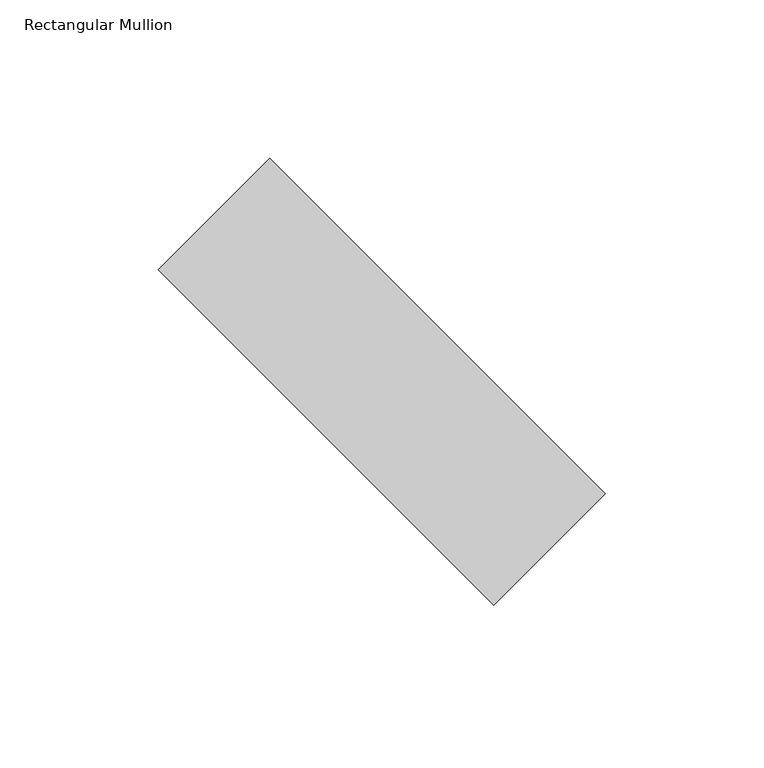
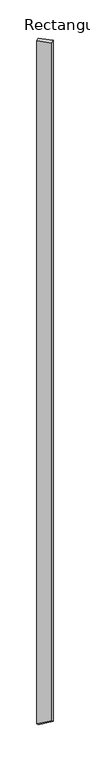
"""IFC4 building model written with IfcOpenShell, lengths in millimetres: member geometry, Rectangular Mullion : tilted mullions."""

import ifcopenshell
import ifcopenshell.guid

model = None  # the IFC model being written
_history = None  # IfcOwnerHistory: only IFC2X3 demands one
_inside = {}  # id of a spatial element -> (the spatial element, [elements in it])
_under = {}  # id of a project, library or spatial element -> (it, [spatial elements below it])
_declared = {}  # id of a project -> (the project, [libraries it declares])
_typed = {}  # id of a type object -> (the type object, [elements of that type])
_made_of = {}  # id of a material, layer set ... -> (it, [elements and type objects made of it])


def new_model(schema):
    """Start an empty IFC model of exactly this schema.

    Asked for "IFC4X3", IfcOpenShell would pick the latest addendum, in which some entities
    have other attributes; the version numbers below select the first issue.
    IFC2X3 requires an IfcOwnerHistory on every rooted entity: one is made here for all.
    """
    global model, _history
    if schema == "IFC4X3":
        model = ifcopenshell.file(schema_version=(4, 3, 0, 0))
    else:
        model = ifcopenshell.file(schema=schema)
    _inside.clear()
    _under.clear()
    _declared.clear()
    _typed.clear()
    _made_of.clear()
    _history = None
    if model.schema == "IFC2X3":
        org = make("IfcOrganization", Name="unknown")
        user = make(
            "IfcPersonAndOrganization",
            ThePerson=make("IfcPerson", FamilyName="unknown"),
            TheOrganization=org,
        )
        app = make(
            "IfcApplication",
            ApplicationDeveloper=org,
            Version="unknown",
            ApplicationFullName="unknown",
            ApplicationIdentifier="unknown",
        )
        _history = make(
            "IfcOwnerHistory",
            OwningUser=user,
            OwningApplication=app,
            ChangeAction="ADDED",
            CreationDate=0,
        )
    return model


def make(cls, **values):
    """One entity of the class cls with the attributes given. An attribute that is None is left unset."""
    return model.create_entity(
        cls, **{name: value for name, value in values.items() if value is not None}
    )


def rooted(cls, **values):
    """An entity with a GlobalId (a new one), such as an element, a storey or a relation."""
    return make(cls, GlobalId=ifcopenshell.guid.new(), OwnerHistory=_history, **values)


def si_unit(unit_type, name, prefix=None):
    """IfcSIUnit, for example si_unit("LENGTHUNIT", "METRE", prefix="MILLI")."""
    return make("IfcSIUnit", UnitType=unit_type, Prefix=prefix, Name=name)


def assignment(units):
    """IfcUnitAssignment: the units of a project."""
    return None if units is None else make("IfcUnitAssignment", Units=units)


def point(xyz):
    """IfcCartesianPoint."""
    return None if xyz is None else make("IfcCartesianPoint", Coordinates=xyz)


def direction(xyz):
    """IfcDirection."""
    return None if xyz is None else make("IfcDirection", DirectionRatios=xyz)


def frame(location, z_axis=None, x_axis=None):
    """IfcAxis2Placement3D, a coordinate frame: its origin and axes. An axis left out is left unset."""
    return make(
        "IfcAxis2Placement3D",
        Location=point(location),
        Axis=direction(z_axis),
        RefDirection=direction(x_axis),
    )


def origin():
    """The frame at (0, 0, 0) with its axes left unset."""
    return frame((0.0, 0.0, 0.0))


def place(relative_to, where):
    """IfcLocalPlacement: puts the frame where relative to a parent placement (None: the world)."""
    return make(
        "IfcLocalPlacement", PlacementRelTo=relative_to, RelativePlacement=where
    )


def context(
    kind, dimensions, precision=None, world=None, true_north=None, identifier=None
):
    """IfcGeometricRepresentationContext, for example the 3D "Model" context."""
    return make(
        "IfcGeometricRepresentationContext",
        ContextIdentifier=identifier,
        ContextType=kind,
        CoordinateSpaceDimension=dimensions,
        Precision=precision,
        WorldCoordinateSystem=world,
        TrueNorth=true_north,
    )


def project(units=None, contexts=None):
    """IfcProject with its units and contexts."""
    return rooted(
        "IfcProject",
        Name="project",
        RepresentationContexts=contexts,
        UnitsInContext=assignment(units),
    )


def spatial(cls, under=None, at=None, **own):
    """A site, building, storey or space (cls), placed at a placement, below another one or the project."""
    s = rooted(cls, ObjectPlacement=at, **own)
    if under is not None:
        _under.setdefault(under.id(), (under, []))[1].append(s)
    return s


def faces_of(points, faces, orient=None, outer=None):
    """IfcFace entities. A face is a list of loops; a loop is a list of indices into points, from 0.

    orient and outer hold one flag for each loop. By default every Orientation is true, the
    first loop of a face is its IfcFaceOuterBound and the others are IfcFaceBound.
    """
    made = []
    for i, loops in enumerate(faces):
        bounds = []
        for j, loop in enumerate(loops):
            is_outer = j == 0 if outer is None else outer[i][j]
            bounds.append(
                make(
                    "IfcFaceOuterBound" if is_outer else "IfcFaceBound",
                    Bound=make("IfcPolyLoop", Polygon=[points[k] for k in loop]),
                    Orientation=True if orient is None else orient[i][j],
                )
            )
        made.append(make("IfcFace", Bounds=bounds))
    return made


def faceted_brep(points, faces, orient=None, outer=None, voids=None):
    """IfcFacetedBrep: a solid bounded by flat faces; with voids (closed shells), ...WithVoids."""
    shared = [point(p) for p in points]
    hull = make("IfcClosedShell", CfsFaces=faces_of(shared, faces, orient, outer))
    if voids is None:
        return make("IfcFacetedBrep", Outer=hull)
    return make(
        "IfcFacetedBrepWithVoids",
        Outer=hull,
        Voids=[
            make(cls, CfsFaces=faces_of(shared, fs, o, b)) for cls, fs, o, b in voids
        ],
    )


def shape(context_of_items, identifier, shape_type, items):
    """IfcShapeRepresentation: the items that make up one representation, for example the "Body"."""
    return make(
        "IfcShapeRepresentation",
        ContextOfItems=context_of_items,
        RepresentationIdentifier=identifier,
        RepresentationType=shape_type,
        Items=items,
    )


def source(mapping_origin, context_of_items, identifier, shape_type, items):
    """IfcRepresentationMap: a shape defined once, which mapped items show again and again."""
    return make(
        "IfcRepresentationMap",
        MappingOrigin=mapping_origin,
        MappedRepresentation=shape(context_of_items, identifier, shape_type, items),
    )


def transform(
    local_origin,
    x_axis=None,
    y_axis=None,
    z_axis=None,
    scale=None,
    scale2=None,
    scale3=None,
    uniform=True,
):
    """IfcCartesianTransformationOperator3D, or its non-uniform kind. x_axis, y_axis, z_axis: its Axis1, 2, 3."""
    if uniform:
        return make(
            "IfcCartesianTransformationOperator3D",
            Axis1=direction(x_axis),
            Axis2=direction(y_axis),
            LocalOrigin=point(local_origin),
            Scale=scale,
            Axis3=direction(z_axis),
        )
    return make(
        "IfcCartesianTransformationOperator3DnonUniform",
        Axis1=direction(x_axis),
        Axis2=direction(y_axis),
        LocalOrigin=point(local_origin),
        Scale=scale,
        Axis3=direction(z_axis),
        Scale2=scale2,
        Scale3=scale3,
    )


def mapped(mapping_source, mapping_target):
    """IfcMappedItem: shows the shape of a source again, moved by a transform."""
    return make(
        "IfcMappedItem", MappingSource=mapping_source, MappingTarget=mapping_target
    )


def made_of(thing, what):
    """Note that an element or type object is made of a material, layer set ...; save() writes the relation."""
    if what is not None:
        _made_of.setdefault(what.id(), (what, []))[1].append(thing)
    return thing


def element(
    cls,
    number,
    at=None,
    inside=None,
    cuts=None,
    type_object=None,
    material=None,
    context=None,
    identifier="Body",
    shape_type=None,
    held_by="IfcProductDefinitionShape",
    body=None,
    shapes=None,
    **own,
):
    """One element of the class cls, such as IfcWall. Its Tag is "e" and its number.

    at: its placement. inside: the storey or other place that contains it. cuts: it is an
    opening in that element (IfcRelVoidsElement). A single representation is given by context,
    identifier, shape_type and body (its items); several are given by shapes. held_by: the class
    of the entity that holds the representations. save() writes the other relations.
    """
    e = rooted(cls, Tag="e%d" % number, ObjectPlacement=at, **own)
    if body is not None:
        shapes = [shape(context, identifier, shape_type, body)]
    if shapes is not None:
        e.Representation = make(held_by, Representations=shapes)
    if inside is not None:
        _inside.setdefault(inside.id(), (inside, []))[1].append(e)
    if cuts is not None:
        rooted(
            "IfcRelVoidsElement", RelatingBuildingElement=cuts, RelatedOpeningElement=e
        )
    if type_object is not None:
        _typed.setdefault(type_object.id(), (type_object, []))[1].append(e)
    return made_of(e, material)


def aggregate(whole, parts):
    """IfcRelAggregates: a whole, such as a stair, and the parts it consists of."""
    return rooted("IfcRelAggregates", RelatingObject=whole, RelatedObjects=parts)


def save(model, path):
    """Write the relations noted so far, then the file.

    IfcRelAggregates (storeys below a building ...), IfcRelContainedInSpatialStructure (elements
    in a storey), IfcRelDefinesByType, IfcRelAssociatesMaterial and IfcRelDeclares: one each for
    every whole, place, type object, material and project.
    """
    for whole, parts in _under.values():
        aggregate(whole, parts)
    for where, things in _inside.values():
        rooted(
            "IfcRelContainedInSpatialStructure",
            RelatedElements=things,
            RelatingStructure=where,
        )
    for kind, things in _typed.values():
        rooted("IfcRelDefinesByType", RelatedObjects=things, RelatingType=kind)
    for what, things in _made_of.values():
        rooted("IfcRelAssociatesMaterial", RelatedObjects=things, RelatingMaterial=what)
    for by, libraries in _declared.values():
        rooted("IfcRelDeclares", RelatingContext=by, RelatedDefinitions=libraries)
    model.write(path)


def rectangular_mullion_71da9a33(model_context):
    return source(origin(), model_context, "Body", "Brep", [
        faceted_brep([(-35.3553391, 70.7106781, 0.0), (-70.7106781, 35.3553391, 0.0), (35.3553391, -70.7106781, 0.0), (70.7106781, -35.3553391, 0.0), (-35.3553391, 70.7106781, -8054.4890214), (-70.7106781, 35.3553391, -8009.469781), (35.3553391, -70.7106781, -7944.2056108), (70.7106781, -35.3553391, -7989.2248513)], [[[0, 1, 2, 3]], [[1, 0, 4, 5]], [[2, 1, 5, 6]], [[3, 2, 6, 7]], [[0, 3, 7, 4]], [[4, 7, 6, 5]]]),
    ])


if __name__ == "__main__":
    model = new_model("IFC4")
    model_context = context("Model", 3, world=origin())
    ifc_project = project(units=[si_unit("LENGTHUNIT", "METRE", prefix="MILLI")], contexts=[model_context])
    site = spatial("IfcSite", under=ifc_project)
    building = spatial("IfcBuilding", under=site)
    placement = place(None, origin())
    rectangular_mullion_shape = rectangular_mullion_71da9a33(model_context)
    element("IfcMember", 1, ObjectType="Rectangular Mullion : tilted mullions", at=placement, inside=building, context=model_context, shape_type="MappedRepresentation", body=[
        mapped(rectangular_mullion_shape, transform((0.0, 0.0, 0.0), x_axis=(1.0, 0.0, 0.0), y_axis=(0.0, 1.0, 0.0), z_axis=(0.0, 0.0, 1.0))),
    ])
    save(model, "model.ifc")

# Revit data of these elements
# Type "Rectangular Mullion : tilted mullions"
#   built-in parameter 1007304 = 0.492126 (stored number, unit not read)
#   built-in parameter 1007301 = 0.082021 (stored number, unit not read)
#   built-in parameter 1007300 = 0.082021 (stored number, unit not read)
# Element 1 (IfcMember, "Rectangular Mullion : tilted mullions")
#   Materials on its faces: "Aluminum"
# Materials
#   "Aluminum": class "Metal", colour RGB 244 244 244, transparency 0, Description = "Aluminum 6061", Cost = 0
